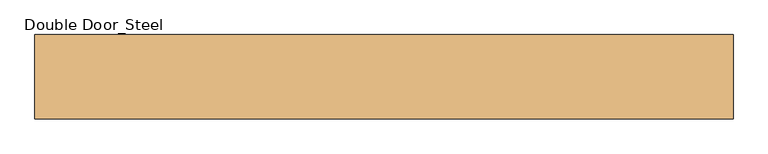
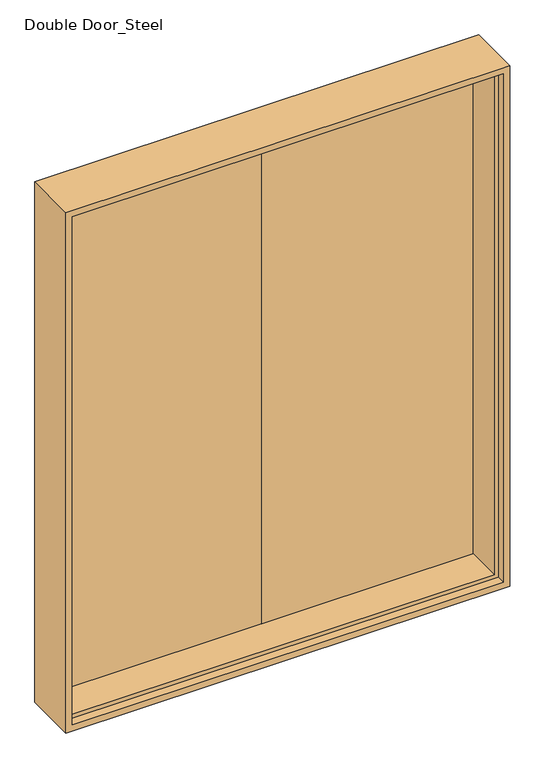
"""IFC4 building model written with IfcOpenShell, lengths in millimetres: door geometry, Double Door_Steel : H_DR_AR B12_Door_Double_W2100xH2580_No FR_SD-5."""

from ifc_helpers import new_model, si_unit, frame, origin, place, context, project, spatial, polyline, outline, extrude, faceted_brep, source, transform, mapped, element, save


def double_door_steel_c24d22a6(model_context):
    return source(origin(), model_context, "Body", "SolidModel", [
        faceted_brep([(-1035.0, -125.0, 2565.0), (-1035.0, 125.0, 2565.0), (-1035.0, 125.0, 0.0), (-1035.0, -125.0, 0.0), (1035.0, 125.0, 0.0), (1035.0, 125.0, 2565.0), (1005.0, 125.0, 2535.0), (-1005.0, 125.0, 2535.0), (-1005.0, 125.0, 30.0), (1005.0, 125.0, 30.0), (1035.0, -125.0, 0.0), (1035.0, -125.0, 2565.0), (1005.0, -125.0, 30.0), (-1005.0, -125.0, 30.0), (-1005.0, -125.0, 2535.0), (1005.0, -125.0, 2535.0), (-1005.0, -85.0, 2535.0), (-1005.0, -85.0, 30.0), (1005.0, -85.0, 30.0), (1005.0, -85.0, 2535.0), (985.0, -85.0, 2515.0), (985.0, -85.0, 50.0), (-985.0, -85.0, 50.0), (-985.0, -85.0, 2515.0), (-985.0, 85.0, 2515.0), (-985.0, 85.0, 50.0), (985.0, 85.0, 50.0), (1005.0, 85.0, 30.0), (-1005.0, 85.0, 30.0), (-1005.0, 85.0, 2535.0), (1005.0, 85.0, 2535.0), (985.0, 85.0, 2515.0)], [[[0, 1, 2, 3]], [[4, 2, 1, 5], [6, 7, 8, 9]], [[3, 2, 4, 10]], [[11, 0, 3, 10], [12, 13, 14, 15]], [[16, 14, 13, 17]], [[17, 13, 12, 18]], [[16, 17, 18, 19], [20, 21, 22, 23]], [[24, 23, 22, 25]], [[25, 22, 21, 26]], [[27, 28, 29, 30], [31, 24, 25, 26]], [[7, 29, 28, 8]], [[8, 28, 27, 9]], [[10, 4, 5, 11]], [[9, 27, 30, 6]], [[18, 12, 15, 19]], [[26, 21, 20, 31]], [[11, 5, 1, 0]], [[19, 15, 14, 16]], [[31, 20, 23, 24]], [[6, 30, 29, 7]]]),
        extrude(outline(polyline([(1005.0, 85.0), (0.0, 85.0), (0.0, 125.0), (1005.0, 125.0), (1005.0, 85.0)])), frame((0.0, 0.0, 30.0), z_axis=(0.0, 0.0, 1.0), x_axis=(1.0, 0.0, 0.0)), (0.0, 0.0, 1.0), 2505.0),
        extrude(outline(polyline([(0.0, 85.0), (-1005.0, 85.0), (-1005.0, 125.0), (0.0, 125.0), (0.0, 85.0)])), frame((0.0, 0.0, 30.0), z_axis=(0.0, 0.0, 1.0), x_axis=(1.0, 0.0, 0.0)), (0.0, 0.0, 1.0), 2505.0),
    ])


if __name__ == "__main__":
    model = new_model("IFC4")
    model_context = context("Model", 3, world=origin())
    ifc_project = project(units=[si_unit("LENGTHUNIT", "METRE", prefix="MILLI")], contexts=[model_context])
    site = spatial("IfcSite", under=ifc_project)
    building = spatial("IfcBuilding", under=site)
    placement = place(None, origin())
    double_door_steel_shape = double_door_steel_c24d22a6(model_context)
    element("IfcDoor", 1, ObjectType="Double Door_Steel : H_DR_AR B12_Door_Double_W2100xH2580_No FR_SD-5", at=placement, inside=building, context=model_context, shape_type="MappedRepresentation", body=[
        mapped(double_door_steel_shape, transform((0.0, 0.0, 0.0), x_axis=(1.0, 0.0, 0.0), y_axis=(0.0, 1.0, 0.0), z_axis=(0.0, 0.0, 1.0))),
    ])
    save(model, "model.ifc")

# Revit data of these elements
# Type "Double Door_Steel : H_DR_AR B12_Door_Double_W2100xH2580_No FR_SD-5"
#   Type Mark = "444"
#   프레임 = ""
#   철물 = ""
#   유리/마감 = ""
#   위치/개소 = ""
#   부호 = ""
#   문번호 = ""
#   문기호 = "SD-5"
#   Analytic Construction = "<None>"
#   Door Width = 1005 mm
#   Height = 2580 mm
#   Width = 2100 mm
#   Define Thermal Properties by = 1
#   문 틀 = none
#   문 = none
#   Function = (empty or 0)
#   Assembly Code = ""
#   Wall Closure = (empty or 0)
